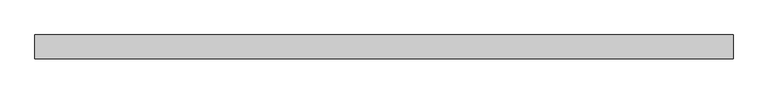
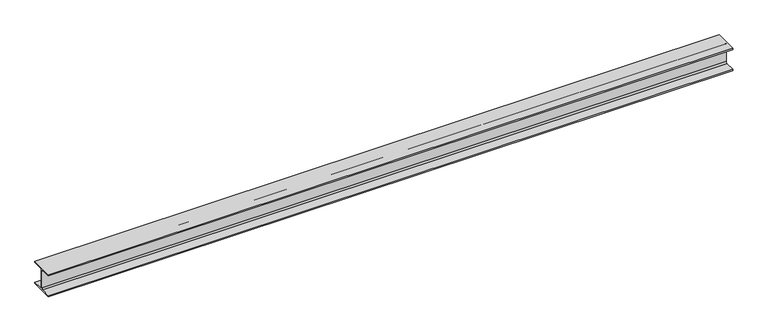
"""IFC4 building model written with IfcOpenShell, lengths in millimetres: beam geometry, 0912_Steel Framing_H-KSD3502 : H_SB_ASB_H-200x200x8x12."""

from ifc_helpers import new_model, si_unit, point, frame, frame_2d, origin, place, context, project, spatial, polyline, circle_curve, trimmed, segment, composite_curve, outline, extrude, source, transform, mapped, element, save


def beam_c011c040(model_context):
    return source(origin(), model_context, "Body", "SweptSolid", [
        extrude(outline(composite_curve([segment(polyline([(100.0, -88.0), (100.0, -100.0), (-100.0, -100.0), (-100.0, -88.0), (-17.0, -88.0)]), True, "CONTINUOUS"), segment(trimmed(circle_curve(frame_2d((-17.0, -75.0)), 13.0), [point((-17.0, -88.0))], [point((-4.0, -75.0))], True, "CARTESIAN"), True, "CONTINUOUS"), segment(polyline([(-4.0, -75.0), (-4.0, 75.0)]), True, "CONTINUOUS"), segment(trimmed(circle_curve(frame_2d((-17.0, 75.0)), 13.0), [point((-4.0, 75.0))], [point((-17.0, 88.0))], True, "CARTESIAN"), True, "CONTINUOUS"), segment(polyline([(-17.0, 88.0), (-100.0, 88.0), (-100.0, 100.0), (100.0, 100.0), (100.0, 88.0), (17.0, 88.0)]), True, "CONTINUOUS"), segment(trimmed(circle_curve(frame_2d((17.0, 75.0)), 13.0), [point((17.0, 88.0))], [point((4.0, 75.0))], True, "CARTESIAN"), True, "CONTINUOUS"), segment(polyline([(4.0, 75.0), (4.0, -75.0)]), True, "CONTINUOUS"), segment(trimmed(circle_curve(frame_2d((17.0, -75.0)), 13.0), [point((4.0, -75.0))], [point((17.0, -88.0))], True, "CARTESIAN"), True, "CONTINUOUS"), segment(polyline([(17.0, -88.0), (100.0, -88.0)]), True, "CONTINUOUS")], self_intersect=False)), frame((-3108.0679819, 0.0, 0.0), z_axis=(1.0, 0.0, 0.0), x_axis=(0.0, 1.0, 0.0)), (0.0, 0.0, 1.0), 5816.9163649),
    ])


if __name__ == "__main__":
    model = new_model("IFC4")
    model_context = context("Model", 3, world=origin())
    ifc_project = project(units=[si_unit("LENGTHUNIT", "METRE", prefix="MILLI")], contexts=[model_context])
    site = spatial("IfcSite", under=ifc_project)
    building = spatial("IfcBuilding", under=site)
    placement = place(None, origin())
    beam_shape = beam_c011c040(model_context)
    element("IfcBeam", 1, ObjectType="0912_Steel Framing_H-KSD3502 : H_SB_ASB_H-200x200x8x12", at=placement, inside=building, context=model_context, shape_type="MappedRepresentation", body=[
        mapped(beam_shape, transform((0.0, 0.0, 0.0), x_axis=(1.0, 0.0, 0.0), y_axis=(0.0, 1.0, 0.0), z_axis=(0.0, 0.0, 1.0))),
    ])
    save(model, "model.ifc")

# Revit data of these elements
# Type "0912_Steel Framing_H-KSD3502 : H_SB_ASB_H-200x200x8x12"
#   H_WM Code_1 = "S01AA002-00001 | Main Steel Structure Fabrication Work | Shelter/Building | Medium Steel - Standard (90KG/M>Weight≥30KG/M) | Material: (   )"
#   H_WM Code_2 = "S03AA028-00001 | Main Steel Structure Erection Work | Shelter/Building | Medium Steel (90KG/M>Weight≥30KG/M) | Material: (   )"
#   H_WM Code_3 = "S01AA010-00001 | Main Steel Structure Fabrication Work | Shelter/Building | Steel Painting/Coating | for Non-Fireproofed Steel Surface, Surface Preparation, Primer, Second & Final Coat | Material: (   )"
#   H_Q'ty Cal Type Tag = "SB-Q2"
#   Width = 20.0 cm
#   Web Thickness = 0.8 cm
#   Web Fillet = 1.3 cm
#   Warping Constant = 141000.0 cm⁶
#   W = 0
#   Torsional Moment of Inertia = 26.2485 cm⁴
#   Section Area = 63.53 cm²
#   Plastic Modulus weak axis = 244.0 cm³
#   Plastic Modulus strong axis = 525.0 cm³
#   Perimeter = 1.16 m²/m
#   Nominal Weight = 49.90 kgf/m
#   Moment of Inertia weak axis = 1600.00 cm⁴
#   Moment of Inertia strong axis = 4720.00 cm⁴
#   Height = 20.0 cm
#   Flange Thickness = 1.2 cm
#   Elastic Modulus weak axis = 160.0 cm³
#   Elastic Modulus strong axis = 472.0 cm³
#   Centroid Vertical = 10.0 cm
#   Centroid Horizontal = 10.0 cm
#   Ix = 47200000
#   Length [instance default] = 1.5240 m
#   Zx = 525000
#   b = 0.2000 m
#   h = 0.2000 m
#   r = 0.0130 m
#   s = 0.0080 m
#   t = 0.0120 m
#   A = 0.006353 m²
#   Structural Material [instance default] = Steel, 45-345
#   Assembly Code = ""
# Element 1 (IfcBeam, "0912_Steel Framing_H-KSD3502 : H_SB_ASB_H-200x200x8x12")
#   Structural Material = none
# Materials
#   "Steel, 45-345": class "Metal", colour RGB 189 187 185, transparency 0, Description = "Steel 345 MPa", Cost = 0
